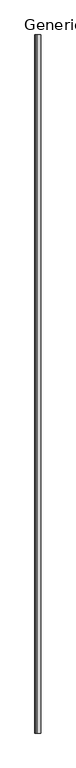
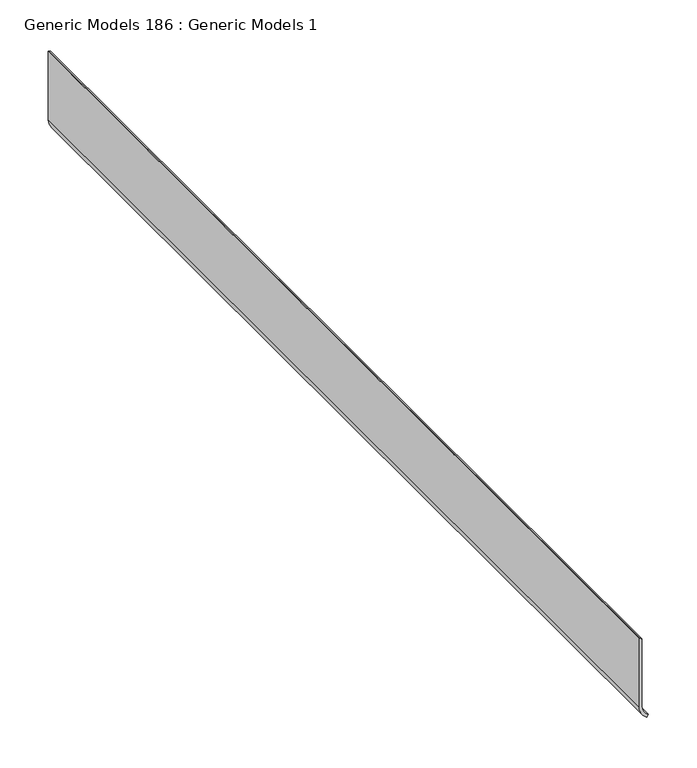
"""IFC4 building model written with IfcOpenShell, lengths in millimetres: proxy geometry, Generic Models 186 : Generic Models 1."""

import ifcopenshell
import ifcopenshell.guid

model = None  # the IFC model being written
_history = None  # IfcOwnerHistory: only IFC2X3 demands one
_inside = {}  # id of a spatial element -> (the spatial element, [elements in it])
_under = {}  # id of a project, library or spatial element -> (it, [spatial elements below it])
_declared = {}  # id of a project -> (the project, [libraries it declares])
_typed = {}  # id of a type object -> (the type object, [elements of that type])
_made_of = {}  # id of a material, layer set ... -> (it, [elements and type objects made of it])


def new_model(schema):
    """Start an empty IFC model of exactly this schema.

    Asked for "IFC4X3", IfcOpenShell would pick the latest addendum, in which some entities
    have other attributes; the version numbers below select the first issue.
    IFC2X3 requires an IfcOwnerHistory on every rooted entity: one is made here for all.
    """
    global model, _history
    if schema == "IFC4X3":
        model = ifcopenshell.file(schema_version=(4, 3, 0, 0))
    else:
        model = ifcopenshell.file(schema=schema)
    _inside.clear()
    _under.clear()
    _declared.clear()
    _typed.clear()
    _made_of.clear()
    _history = None
    if model.schema == "IFC2X3":
        org = make("IfcOrganization", Name="unknown")
        user = make(
            "IfcPersonAndOrganization",
            ThePerson=make("IfcPerson", FamilyName="unknown"),
            TheOrganization=org,
        )
        app = make(
            "IfcApplication",
            ApplicationDeveloper=org,
            Version="unknown",
            ApplicationFullName="unknown",
            ApplicationIdentifier="unknown",
        )
        _history = make(
            "IfcOwnerHistory",
            OwningUser=user,
            OwningApplication=app,
            ChangeAction="ADDED",
            CreationDate=0,
        )
    return model


def make(cls, **values):
    """One entity of the class cls with the attributes given. An attribute that is None is left unset."""
    return model.create_entity(
        cls, **{name: value for name, value in values.items() if value is not None}
    )


def rooted(cls, **values):
    """An entity with a GlobalId (a new one), such as an element, a storey or a relation."""
    return make(cls, GlobalId=ifcopenshell.guid.new(), OwnerHistory=_history, **values)


def si_unit(unit_type, name, prefix=None):
    """IfcSIUnit, for example si_unit("LENGTHUNIT", "METRE", prefix="MILLI")."""
    return make("IfcSIUnit", UnitType=unit_type, Prefix=prefix, Name=name)


def assignment(units):
    """IfcUnitAssignment: the units of a project."""
    return None if units is None else make("IfcUnitAssignment", Units=units)


def point(xyz):
    """IfcCartesianPoint."""
    return None if xyz is None else make("IfcCartesianPoint", Coordinates=xyz)


def direction(xyz):
    """IfcDirection."""
    return None if xyz is None else make("IfcDirection", DirectionRatios=xyz)


def frame(location, z_axis=None, x_axis=None):
    """IfcAxis2Placement3D, a coordinate frame: its origin and axes. An axis left out is left unset."""
    return make(
        "IfcAxis2Placement3D",
        Location=point(location),
        Axis=direction(z_axis),
        RefDirection=direction(x_axis),
    )


def frame_2d(location, x_axis=None):
    """IfcAxis2Placement2D, a coordinate frame in the plane: its origin and x axis."""
    return make(
        "IfcAxis2Placement2D", Location=point(location), RefDirection=direction(x_axis)
    )


def origin():
    """The frame at (0, 0, 0) with its axes left unset."""
    return frame((0.0, 0.0, 0.0))


def place(relative_to, where):
    """IfcLocalPlacement: puts the frame where relative to a parent placement (None: the world)."""
    return make(
        "IfcLocalPlacement", PlacementRelTo=relative_to, RelativePlacement=where
    )


def context(
    kind, dimensions, precision=None, world=None, true_north=None, identifier=None
):
    """IfcGeometricRepresentationContext, for example the 3D "Model" context."""
    return make(
        "IfcGeometricRepresentationContext",
        ContextIdentifier=identifier,
        ContextType=kind,
        CoordinateSpaceDimension=dimensions,
        Precision=precision,
        WorldCoordinateSystem=world,
        TrueNorth=true_north,
    )


def project(units=None, contexts=None):
    """IfcProject with its units and contexts."""
    return rooted(
        "IfcProject",
        Name="project",
        RepresentationContexts=contexts,
        UnitsInContext=assignment(units),
    )


def spatial(cls, under=None, at=None, **own):
    """A site, building, storey or space (cls), placed at a placement, below another one or the project."""
    s = rooted(cls, ObjectPlacement=at, **own)
    if under is not None:
        _under.setdefault(under.id(), (under, []))[1].append(s)
    return s


def polyline(points):
    """IfcPolyline through the points."""
    return make("IfcPolyline", Points=[point(p) for p in points])


def circle_curve(where, radius):
    """IfcCircle in the frame where."""
    return make("IfcCircle", Position=where, Radius=radius)


def trimmed(basis, trim1, trim2, sense, master):
    """IfcTrimmedCurve: the piece of a basis curve between two trims."""
    return make(
        "IfcTrimmedCurve",
        BasisCurve=basis,
        Trim1=trim1,
        Trim2=trim2,
        SenseAgreement=sense,
        MasterRepresentation=master,
    )


def segment(curve, same_sense, transition):
    """IfcCompositeCurveSegment."""
    return make(
        "IfcCompositeCurveSegment",
        Transition=transition,
        SameSense=same_sense,
        ParentCurve=curve,
    )


def composite_curve(segments, self_intersect=None):
    """IfcCompositeCurve: segments joined end to end."""
    return make("IfcCompositeCurve", Segments=segments, SelfIntersect=self_intersect)


def outline(outer, holes=None, kind="AREA"):
    """IfcArbitraryClosedProfileDef: a profile drawn as a closed curve; with holes, ...WithVoids."""
    if holes is None:
        return make("IfcArbitraryClosedProfileDef", ProfileType=kind, OuterCurve=outer)
    return make(
        "IfcArbitraryProfileDefWithVoids",
        ProfileType=kind,
        OuterCurve=outer,
        InnerCurves=holes,
    )


def extrude(swept, where, along, depth):
    """IfcExtrudedAreaSolid: the profile swept, set in the frame where, extruded along a direction by depth."""
    return make(
        "IfcExtrudedAreaSolid",
        SweptArea=swept,
        Position=where,
        ExtrudedDirection=direction(along),
        Depth=depth,
    )


def shape(context_of_items, identifier, shape_type, items):
    """IfcShapeRepresentation: the items that make up one representation, for example the "Body"."""
    return make(
        "IfcShapeRepresentation",
        ContextOfItems=context_of_items,
        RepresentationIdentifier=identifier,
        RepresentationType=shape_type,
        Items=items,
    )


def source(mapping_origin, context_of_items, identifier, shape_type, items):
    """IfcRepresentationMap: a shape defined once, which mapped items show again and again."""
    return make(
        "IfcRepresentationMap",
        MappingOrigin=mapping_origin,
        MappedRepresentation=shape(context_of_items, identifier, shape_type, items),
    )


def transform(
    local_origin,
    x_axis=None,
    y_axis=None,
    z_axis=None,
    scale=None,
    scale2=None,
    scale3=None,
    uniform=True,
):
    """IfcCartesianTransformationOperator3D, or its non-uniform kind. x_axis, y_axis, z_axis: its Axis1, 2, 3."""
    if uniform:
        return make(
            "IfcCartesianTransformationOperator3D",
            Axis1=direction(x_axis),
            Axis2=direction(y_axis),
            LocalOrigin=point(local_origin),
            Scale=scale,
            Axis3=direction(z_axis),
        )
    return make(
        "IfcCartesianTransformationOperator3DnonUniform",
        Axis1=direction(x_axis),
        Axis2=direction(y_axis),
        LocalOrigin=point(local_origin),
        Scale=scale,
        Axis3=direction(z_axis),
        Scale2=scale2,
        Scale3=scale3,
    )


def mapped(mapping_source, mapping_target):
    """IfcMappedItem: shows the shape of a source again, moved by a transform."""
    return make(
        "IfcMappedItem", MappingSource=mapping_source, MappingTarget=mapping_target
    )


def made_of(thing, what):
    """Note that an element or type object is made of a material, layer set ...; save() writes the relation."""
    if what is not None:
        _made_of.setdefault(what.id(), (what, []))[1].append(thing)
    return thing


def element(
    cls,
    number,
    at=None,
    inside=None,
    cuts=None,
    type_object=None,
    material=None,
    context=None,
    identifier="Body",
    shape_type=None,
    held_by="IfcProductDefinitionShape",
    body=None,
    shapes=None,
    **own,
):
    """One element of the class cls, such as IfcWall. Its Tag is "e" and its number.

    at: its placement. inside: the storey or other place that contains it. cuts: it is an
    opening in that element (IfcRelVoidsElement). A single representation is given by context,
    identifier, shape_type and body (its items); several are given by shapes. held_by: the class
    of the entity that holds the representations. save() writes the other relations.
    """
    e = rooted(cls, Tag="e%d" % number, ObjectPlacement=at, **own)
    if body is not None:
        shapes = [shape(context, identifier, shape_type, body)]
    if shapes is not None:
        e.Representation = make(held_by, Representations=shapes)
    if inside is not None:
        _inside.setdefault(inside.id(), (inside, []))[1].append(e)
    if cuts is not None:
        rooted(
            "IfcRelVoidsElement", RelatingBuildingElement=cuts, RelatedOpeningElement=e
        )
    if type_object is not None:
        _typed.setdefault(type_object.id(), (type_object, []))[1].append(e)
    return made_of(e, material)


def aggregate(whole, parts):
    """IfcRelAggregates: a whole, such as a stair, and the parts it consists of."""
    return rooted("IfcRelAggregates", RelatingObject=whole, RelatedObjects=parts)


def save(model, path):
    """Write the relations noted so far, then the file.

    IfcRelAggregates (storeys below a building ...), IfcRelContainedInSpatialStructure (elements
    in a storey), IfcRelDefinesByType, IfcRelAssociatesMaterial and IfcRelDeclares: one each for
    every whole, place, type object, material and project.
    """
    for whole, parts in _under.values():
        aggregate(whole, parts)
    for where, things in _inside.values():
        rooted(
            "IfcRelContainedInSpatialStructure",
            RelatedElements=things,
            RelatingStructure=where,
        )
    for kind, things in _typed.values():
        rooted("IfcRelDefinesByType", RelatedObjects=things, RelatingType=kind)
    for what, things in _made_of.values():
        rooted("IfcRelAssociatesMaterial", RelatedObjects=things, RelatingMaterial=what)
    for by, libraries in _declared.values():
        rooted("IfcRelDeclares", RelatingContext=by, RelatedDefinitions=libraries)
    model.write(path)


def generic_models_186_generic_models_1_ef70466a(model_context):
    return source(origin(), model_context, "Body", "SweptSolid", [
        extrude(outline(composite_curve([segment(polyline([(101.6, 49799.875), (15.4496307, 49799.875)]), True, "CONTINUOUS"), segment(trimmed(circle_curve(frame_2d((15.4496307, 49817.7146968)), 17.8396968), [point((15.4496307, 49799.875))], [point((0.0, 49808.7948484))], False, "CARTESIAN"), True, "CONTINUOUS"), segment(polyline([(0.0, 49808.7948484), (2.7496307, 49810.3823484)]), True, "CONTINUOUS"), segment(trimmed(circle_curve(frame_2d((15.4496307, 49817.7146968)), 14.6646968), [point((2.7496307, 49810.3823484))], [point((15.4496307, 49803.05))], True, "CARTESIAN"), True, "CONTINUOUS"), segment(polyline([(15.4496307, 49803.05), (99.5131982, 49803.05)]), True, "CONTINUOUS"), segment(trimmed(circle_curve(frame_2d((99.5131982, 49800.9631982)), 2.0868018), [point((99.5131982, 49803.05))], [point((101.6, 49800.9631982))], False, "CARTESIAN"), True, "CONTINUOUS"), segment(polyline([(101.6, 49800.9631982), (101.6, 49799.875)]), True, "CONTINUOUS")], self_intersect=False)), frame((0.0, 0.0, 0.0), z_axis=(0.0, 1.0, 0.0), x_axis=(0.0, 0.0, 1.0)), (0.0, 0.0, 1.0), 1219.2),
    ])


if __name__ == "__main__":
    model = new_model("IFC4")
    model_context = context("Model", 3, world=origin())
    ifc_project = project(units=[si_unit("LENGTHUNIT", "METRE", prefix="MILLI")], contexts=[model_context])
    site = spatial("IfcSite", under=ifc_project)
    building = spatial("IfcBuilding", under=site)
    placement = place(None, origin())
    generic_models_186_generic_models_1_shape = generic_models_186_generic_models_1_ef70466a(model_context)
    element("IfcBuildingElementProxy", 1, Name="Generic Models 186 : Generic Models 1", ObjectType="Generic Models 186 : Generic Models 1", at=placement, inside=building, context=model_context, shape_type="MappedRepresentation", body=[
        mapped(generic_models_186_generic_models_1_shape, transform((0.0, 0.0, 0.0), x_axis=(1.0, 0.0, 0.0), y_axis=(0.0, 1.0, 0.0), z_axis=(0.0, 0.0, 1.0))),
    ])
    save(model, "model.ifc")

# Revit data of these elements
# Element 1 (IfcBuildingElementProxy, "Generic Models 186 : Generic Models 1")
#   Materials on its faces: "MATCH EXISTING BASE"
# Materials
#   "MATCH EXISTING BASE": class "Generic", colour RGB 120 120 120, transparency 0, Cost = 0
